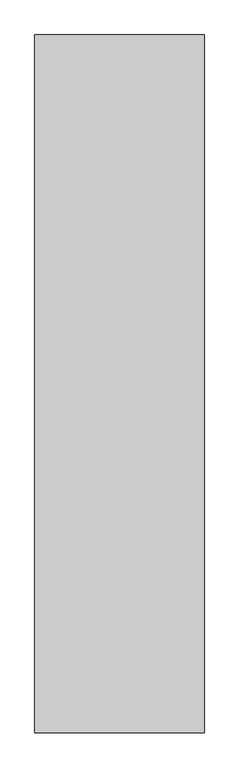
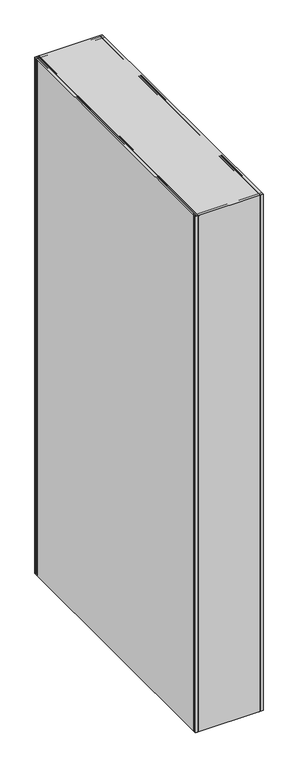
"""IFC4 building model written with IfcOpenShell, lengths in millimetres: beam geometry, LF02ZBK001_DIKE WALL_RC : Dike_Thk.260_EW1."""

from ifc_helpers import new_model, si_unit, origin, origin_with_axes, place, context, project, spatial, polyline, outline, extrude, source, transform, mapped, element, save


def beam_92c4ef8c(model_context):
    return source(origin(), model_context, "Body", "SweptSolid", [
        extrude(outline(polyline([(130.0, -535.0), (-130.0, -535.0), (-130.0, 535.0), (130.0, 535.0), (130.0, -535.0)])), origin_with_axes(), (0.0, 0.0, 1.0), 2100.0),
        extrude(outline(polyline([(-130.0, -520.0), (-130.0, -519.0), (130.0, -519.0), (130.0, -520.0), (-130.0, -520.0)])), origin_with_axes(), (0.0, 0.0, 1.0), 2100.0),
        extrude(outline(polyline([(-130.0, -525.0), (-130.0, -524.0), (130.0, -524.0), (130.0, -525.0), (-130.0, -525.0)])), origin_with_axes(), (0.0, 0.0, 1.0), 2100.0),
        extrude(outline(polyline([(-130.0, -530.0), (-130.0, -529.0), (130.0, -529.0), (130.0, -530.0), (-130.0, -530.0)])), origin_with_axes(), (0.0, 0.0, 1.0), 2100.0),
        extrude(outline(polyline([(-130.0, 520.0), (130.0, 520.0), (130.0, 519.0), (-130.0, 519.0), (-130.0, 520.0)])), origin_with_axes(), (0.0, 0.0, 1.0), 2100.0),
        extrude(outline(polyline([(-130.0, 525.0), (130.0, 525.0), (130.0, 524.0), (-130.0, 524.0), (-130.0, 525.0)])), origin_with_axes(), (0.0, 0.0, 1.0), 2100.0),
        extrude(outline(polyline([(-130.0, 530.0), (130.0, 530.0), (130.0, 529.0), (-130.0, 529.0), (-130.0, 530.0)])), origin_with_axes(), (0.0, 0.0, 1.0), 2100.0),
        extrude(outline(polyline([(114.0, 535.0), (115.0, 535.0), (115.0, -535.0), (114.0, -535.0), (114.0, 535.0)])), origin_with_axes(), (0.0, 0.0, 1.0), 2100.0),
        extrude(outline(polyline([(119.0, 535.0), (120.0, 535.0), (120.0, -535.0), (119.0, -535.0), (119.0, 535.0)])), origin_with_axes(), (0.0, 0.0, 1.0), 2100.0),
        extrude(outline(polyline([(124.0, 535.0), (125.0, 535.0), (125.0, -535.0), (124.0, -535.0), (124.0, 535.0)])), origin_with_axes(), (0.0, 0.0, 1.0), 2100.0),
        extrude(outline(polyline([(-114.0, 535.0), (-114.0, -535.0), (-115.0, -535.0), (-115.0, 535.0), (-114.0, 535.0)])), origin_with_axes(), (0.0, 0.0, 1.0), 2100.0),
        extrude(outline(polyline([(-119.0, 535.0), (-119.0, -535.0), (-120.0, -535.0), (-120.0, 535.0), (-119.0, 535.0)])), origin_with_axes(), (0.0, 0.0, 1.0), 2100.0),
        extrude(outline(polyline([(-124.0, 535.0), (-124.0, -535.0), (-125.0, -535.0), (-125.0, 535.0), (-124.0, 535.0)])), origin_with_axes(), (0.0, 0.0, 1.0), 2100.0),
    ])


if __name__ == "__main__":
    model = new_model("IFC4")
    model_context = context("Model", 3, world=origin())
    ifc_project = project(units=[si_unit("LENGTHUNIT", "METRE", prefix="MILLI")], contexts=[model_context])
    site = spatial("IfcSite", under=ifc_project)
    building = spatial("IfcBuilding", under=site)
    placement = place(None, origin())
    beam_shape = beam_92c4ef8c(model_context)
    element("IfcBeam", 1, ObjectType="LF02ZBK001_DIKE WALL_RC : Dike_Thk.260_EW1", at=placement, inside=building, context=model_context, shape_type="MappedRepresentation", body=[
        mapped(beam_shape, transform((0.0, 0.0, 0.0), x_axis=(1.0, 0.0, 0.0), y_axis=(0.0, 1.0, 0.0), z_axis=(0.0, 0.0, 1.0))),
    ])
    save(model, "model.ifc")

# Revit data of these elements
# Type "LF02ZBK001_DIKE WALL_RC : Dike_Thk.260_EW1"
#   Dike_thk = 260 mm
#   Dike_Length [instance default] = 3000 mm
#   Dike_Hight = 2100 mm
#   c2_visible = yes
#   c3_material [instance default] = none
#   c2_material 3 [instance default] = none
#   c2_material 2 [instance default] = none
#   c2_material 1 [instance default] = none
#   c1_material [instance default] = none
#   Default Elevation = 0
# Element 1 (IfcBeam, "LF02ZBK001_DIKE WALL_RC : Dike_Thk.260_EW1")
#   Dike_Length = 1070 mm
